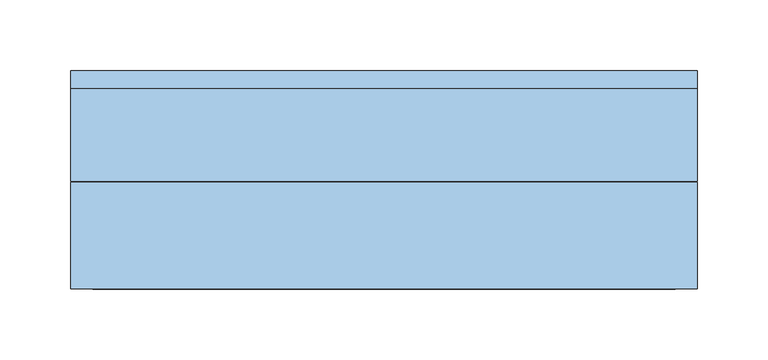
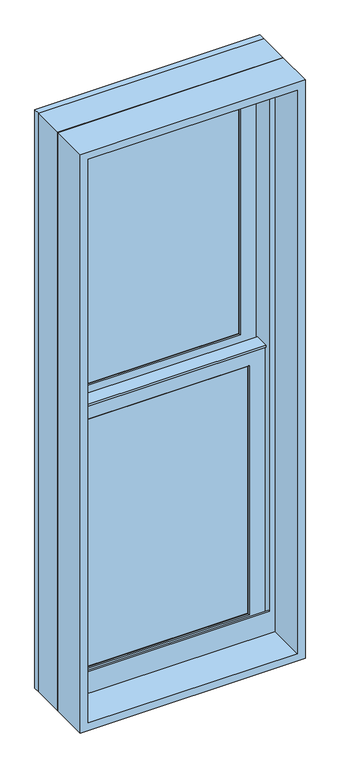
"""IFC4 building model written with IfcOpenShell, lengths in millimetres: window geometry, Window-Double_Hung-Marvin-Essential : ESDH1640."""

from ifc_helpers import new_model, si_unit, frame, origin, place, context, project, spatial, polyline, outline, extrude, faceted_brep, source, transform, mapped, element, save


def window_cbfb7004(model_context):
    return source(origin(), model_context, "Body", "SolidModel", [
        extrude(outline(polyline([(64.5583333, 20.6375), (64.5583333, 15.875), (45.5083333, 15.875), (45.5083333, 20.6375), (64.5583333, 20.6375)])), frame((0.0, 0.0, 1289.05), z_axis=(0.0, 0.0, 1.0), x_axis=(1.0, 0.0, 0.0)), (0.0, 0.0, 1.0), 527.05),
        extrude(outline(polyline([(-45.5083333, 20.6375), (-45.5083333, 15.875), (-64.5583333, 15.875), (-64.5583333, 20.6375), (-45.5083333, 20.6375)])), frame((0.0, 0.0, 1289.05), z_axis=(0.0, 0.0, 1.0), x_axis=(1.0, 0.0, 0.0)), (0.0, 0.0, 1.0), 527.05),
        extrude(outline(polyline([(165.1, 20.6375), (165.1, 15.875), (-165.1, 15.875), (-165.1, 20.6375), (165.1, 20.6375)])), frame((0.0, 0.0, 1543.05), z_axis=(0.0, 0.0, 1.0), x_axis=(1.0, 0.0, 0.0)), (0.0, 0.0, 1.0), 19.05),
        extrude(outline(polyline([(-64.5583333, 46.83125), (-64.5583333, 51.59375), (-45.5083333, 51.59375), (-45.5083333, 46.83125), (-64.5583333, 46.83125)])), frame((0.0, 0.0, 1854.2), z_axis=(0.0, 0.0, 1.0), x_axis=(1.0, 0.0, 0.0)), (0.0, 0.0, 1.0), 527.05),
        extrude(outline(polyline([(45.5083333, 46.83125), (45.5083333, 51.59375), (64.5583333, 51.59375), (64.5583333, 46.83125), (45.5083333, 46.83125)])), frame((0.0, 0.0, 1854.2), z_axis=(0.0, 0.0, 1.0), x_axis=(1.0, 0.0, 0.0)), (0.0, 0.0, 1.0), 527.05),
        extrude(outline(polyline([(-165.1, 46.83125), (-165.1, 51.59375), (165.1, 51.59375), (165.1, 46.83125), (-165.1, 46.83125)])), frame((0.0, 0.0, 2108.2), z_axis=(0.0, 0.0, 1.0), x_axis=(1.0, 0.0, 0.0)), (0.0, 0.0, 1.0), 19.05),
        extrude(outline(polyline([(64.5583333, 20.6375), (45.5083333, 20.6375), (45.5083333, 25.4), (64.5583333, 25.4), (64.5583333, 20.6375)])), frame((0.0, 0.0, 1289.05), z_axis=(0.0, 0.0, 1.0), x_axis=(1.0, 0.0, 0.0)), (0.0, 0.0, 1.0), 527.05),
        extrude(outline(polyline([(-45.5083333, 20.6375), (-64.5583333, 20.6375), (-64.5583333, 25.4), (-45.5083333, 25.4), (-45.5083333, 20.6375)])), frame((0.0, 0.0, 1289.05), z_axis=(0.0, 0.0, 1.0), x_axis=(1.0, 0.0, 0.0)), (0.0, 0.0, 1.0), 527.05),
        extrude(outline(polyline([(165.1, 20.6375), (-165.1, 20.6375), (-165.1, 25.4), (165.1, 25.4), (165.1, 20.6375)])), frame((0.0, 0.0, 1543.05), z_axis=(0.0, 0.0, 1.0), x_axis=(1.0, 0.0, 0.0)), (0.0, 0.0, 1.0), 19.05),
        extrude(outline(polyline([(-64.5583333, 56.35625), (-45.5083333, 56.35625), (-45.5083333, 51.59375), (-64.5583333, 51.59375), (-64.5583333, 56.35625)])), frame((0.0, 0.0, 1854.2), z_axis=(0.0, 0.0, 1.0), x_axis=(1.0, 0.0, 0.0)), (0.0, 0.0, 1.0), 527.05),
        extrude(outline(polyline([(45.5083333, 56.35625), (64.5583333, 56.35625), (64.5583333, 51.59375), (45.5083333, 51.59375), (45.5083333, 56.35625)])), frame((0.0, 0.0, 1854.2), z_axis=(0.0, 0.0, 1.0), x_axis=(1.0, 0.0, 0.0)), (0.0, 0.0, 1.0), 527.05),
        extrude(outline(polyline([(-165.1, 56.35625), (165.1, 56.35625), (165.1, 51.59375), (-165.1, 51.59375), (-165.1, 56.35625)])), frame((0.0, 0.0, 2108.2), z_axis=(0.0, 0.0, 1.0), x_axis=(1.0, 0.0, 0.0)), (0.0, 0.0, 1.0), 19.05),
        faceted_brep([(-192.0875, 5.6780605, 1846.1351748), (-192.0875, 5.6780605, 1841.5), (192.0875, 5.6780605, 1841.5), (192.0875, 5.6780605, 1846.1351748), (-192.0875, 34.8118605, 1846.1351748), (192.0875, 34.8118605, 1846.1351748), (192.0875, 34.8118605, 1841.5), (-192.0875, 34.8118605, 1841.5), (-192.0875, 30.1625, 1841.5), (-192.0875, 30.1625, 1262.0625), (-192.0875, 8.9241104, 1262.0625), (-192.0875, 8.9241104, 1841.5), (192.0875, 8.9241104, 1841.5), (192.0875, 30.1625, 1841.5), (192.0875, 8.9241104, 1262.0625), (192.0875, 30.1625, 1262.0625), (-176.2034752, 11.90625, 1827.2034752), (-176.2034752, 30.1625, 1827.2034752), (176.2034752, 30.1625, 1827.2034752), (176.2034752, 11.90625, 1827.2034752), (-159.54375, 10.4662439, 1810.54375), (-159.54375, 11.90625, 1810.54375), (159.54375, 11.90625, 1810.54375), (159.54375, 10.4662439, 1810.54375), (161.0858834, 8.9241104, 1812.0858834), (-161.0858834, 8.9241104, 1812.0858834), (176.2034752, 30.1625, 1277.9465248), (176.2034752, 11.90625, 1277.9465248), (159.54375, 11.90625, 1294.60625), (159.54375, 10.4662439, 1294.60625), (161.0858834, 8.9241104, 1293.0641166), (-176.2034752, 30.1625, 1277.9465248), (-176.2034752, 11.90625, 1277.9465248), (-159.54375, 11.90625, 1294.60625), (-159.54375, 10.4662439, 1294.60625), (-161.0858834, 8.9241104, 1293.0641166)], [[[0, 1, 2, 3]], [[4, 5, 6, 7]], [[1, 0, 4, 7, 8, 9, 10, 11]], [[2, 1, 11, 12]], [[7, 6, 13, 8]], [[3, 2, 12, 14, 15, 13, 6, 5]], [[0, 3, 5, 4]], [[16, 17, 18, 19]], [[20, 21, 22, 23]], [[20, 23, 24, 25]], [[19, 18, 26, 27]], [[23, 22, 28, 29]], [[24, 23, 29, 30]], [[27, 26, 31, 32]], [[29, 28, 33, 34]], [[30, 29, 34, 35]], [[15, 14, 10, 9]], [[15, 9, 8, 13], [18, 17, 31, 26]], [[17, 16, 32, 31]], [[16, 19, 27, 32], [22, 21, 33, 28]], [[21, 20, 34, 33]], [[20, 25, 35, 34]], [[10, 14, 12, 11], [25, 24, 30, 35]]]),
        extrude(outline(polyline([(38.5955581, 1827.2125), (33.5778968, 1827.2125), (33.5778968, 1828.8), (39.9405976, 1828.8), (39.9405976, 1827.2125), (61.515625, 1827.2125), (47.6307501, 1823.8975159), (38.5955581, 1823.8975159), (38.5955581, 1827.2125)])), frame((-192.0875, 0.0, 0.0), z_axis=(1.0, 0.0, 0.0), x_axis=(0.0, 1.0, 0.0)), (0.0, 0.0, 1.0), 384.175),
        faceted_brep([(222.25, 0.0, 1231.9), (222.25, 0.0, 2438.4), (-222.25, 0.0, 2438.4), (-222.25, 0.0, 1231.9), (196.05625, 0.0, 1293.01875), (-196.05625, 0.0, 1293.01875), (-196.05625, 0.0, 2412.20625), (196.05625, 0.0, 2412.20625), (196.05625, 3.96875, 1231.9), (-196.05625, 3.96875, 1231.9), (-196.05625, 3.96875, 1293.01875), (196.05625, 3.96875, 1293.01875), (-222.25, 65.6828125, 1231.9), (-196.05625, 65.6828125, 1231.9), (196.05625, 65.6828125, 1231.9), (222.25, 65.6828125, 1231.9), (-222.25, 65.6828125, 2438.4), (222.25, 65.6828125, 2438.4), (196.05625, 65.6828125, 2412.20625), (-196.05625, 65.6828125, 2412.20625)], [[[0, 1, 2, 3], [4, 5, 6, 7]], [[8, 9, 10, 11]], [[5, 4, 11, 10]], [[0, 3, 12, 13, 9, 8, 14, 15]], [[13, 12, 16, 17, 15, 14, 18, 19]], [[13, 19, 6, 5, 10, 9]], [[7, 6, 19, 18]], [[18, 14, 8, 11, 4, 7]], [[1, 0, 15, 17]], [[2, 1, 17, 16]], [[3, 2, 16, 12]]]),
        faceted_brep([(196.05625, 30.1625, 1835.15), (194.46875, 30.1625, 1835.15), (194.46875, 30.1625, 1256.2544613), (196.05625, 30.1625, 1256.2544613), (-194.46875, 30.1625, 1835.15), (-196.05625, 30.1625, 1835.15), (-196.05625, 30.1625, 1256.2544613), (-194.46875, 30.1625, 1256.2544613), (194.46875, 63.5, 1835.15), (196.05625, 63.5, 1835.15), (196.05625, 63.5, 1249.7743077), (194.46875, 63.5, 1249.7743077), (-196.05625, 63.5, 1835.15), (-194.46875, 63.5, 1835.15), (-194.46875, 63.5, 1249.7743077), (-196.05625, 63.5, 1249.7743077), (207.3108932, 3.96875, 1261.3460105), (207.3108932, 3.96875, 1231.9), (207.3108932, 65.6828125, 1231.9), (207.3108932, 65.6828125, 1249.350012), (-207.3108932, 3.96875, 1231.9), (-207.3108932, 3.96875, 1261.3460105), (-207.3108932, 65.6828125, 1249.350012), (-207.3108932, 65.6828125, 1231.9), (207.3108932, 78.58125, 1246.8428097), (-207.3108932, 78.58125, 1246.8428097), (-205.2971252, 68.2348864, 1248.8539391), (-187.33135, 68.2348864, 1248.8539391), (-187.33135, 65.6828125, 1249.350012), (187.33135, 65.6828125, 1249.350012), (187.33135, 68.2348864, 1248.8539391), (205.2971252, 68.2348864, 1248.8539391), (-222.25, 65.6828125, 1231.9), (-222.25, 78.5948249, 1231.9), (222.25, 78.5948249, 1231.9), (222.25, 65.6828125, 1231.9), (-222.25, 78.58125, 2438.4), (222.25, 78.58125, 2438.4), (207.3108932, 78.58125, 2423.4608932), (-207.3108932, 78.58125, 2423.4608932), (-222.25, 65.6828125, 2438.4), (-205.2971252, 68.2348864, 2421.4471252), (205.2971252, 68.2348864, 2421.4471252), (187.33135, 68.2348864, 2403.48135), (-187.33135, 68.2348864, 2403.48135), (-187.33135, 65.6828125, 2403.48135), (187.33135, 65.6828125, 2403.48135), (222.25, 65.6828125, 2438.4)], [[[0, 1, 2, 3]], [[4, 5, 6, 7]], [[8, 9, 10, 11]], [[12, 13, 14, 15]], [[1, 8, 11, 2]], [[9, 0, 3, 10]], [[1, 0, 9, 8]], [[5, 4, 13, 12]], [[5, 12, 15, 6]], [[13, 4, 7, 14]], [[16, 17, 18, 19]], [[20, 21, 22, 23]], [[24, 25, 26, 27, 28, 22, 21, 16, 19, 29, 30, 31], [3, 2, 11, 10], [7, 6, 15, 14]], [[17, 16, 21, 20]], [[17, 20, 23, 32, 33, 34, 35, 18]], [[34, 33, 36, 37], [25, 24, 38, 39]], [[33, 32, 40, 36]], [[39, 41, 26, 25]], [[41, 42, 31, 30, 43, 44, 27, 26]], [[44, 45, 28, 27]], [[40, 32, 23, 22, 28, 45, 46, 29, 19, 18, 35, 47]], [[36, 40, 47, 37]], [[39, 38, 42, 41]], [[44, 43, 46, 45]], [[34, 37, 47, 35]], [[42, 38, 24, 31]], [[46, 43, 30, 29]]]),
        extrude(outline(polyline([(172.24375, 11.90625), (-172.24375, 11.90625), (-172.24375, 15.08125), (172.24375, 15.08125), (172.24375, 11.90625)])), frame((0.0, 0.0, 1281.90625), z_axis=(0.0, 0.0, 1.0), x_axis=(1.0, 0.0, 0.0)), (0.0, 0.0, 1.0), 541.3375),
        extrude(outline(polyline([(172.24375, 42.8625), (-172.24375, 42.8625), (-172.24375, 46.0375), (172.24375, 46.0375), (172.24375, 42.8625)])), frame((0.0, 0.0, 1847.05625), z_axis=(0.0, 0.0, 1.0), x_axis=(1.0, 0.0, 0.0)), (0.0, 0.0, 1.0), 541.3375),
        faceted_brep([(-159.54375, 31.194477, 1810.54375), (-161.0858834, 32.7366104, 1812.0858834), (161.0858834, 32.7366104, 1812.0858834), (159.54375, 31.194477, 1810.54375), (-159.54375, 30.1625, 1810.54375), (159.54375, 30.1625, 1810.54375), (-192.0875, 32.7366104, 1843.0875), (-192.0875, 30.1625, 1843.0875), (192.0875, 30.1625, 1843.0875), (192.0875, 32.7366104, 1843.0875), (161.0858834, 32.7366104, 1293.0641166), (159.54375, 31.194477, 1294.60625), (159.54375, 30.1625, 1294.60625), (192.0875, 30.1625, 1262.0625), (192.0875, 32.7366104, 1262.0625), (-161.0858834, 32.7366104, 1293.0641166), (-159.54375, 31.194477, 1294.60625), (-159.54375, 30.1625, 1294.60625), (-192.0875, 30.1625, 1262.0625), (-192.0875, 32.7366104, 1262.0625)], [[[0, 1, 2, 3]], [[4, 0, 3, 5]], [[6, 7, 8, 9]], [[3, 2, 10, 11]], [[5, 3, 11, 12]], [[9, 8, 13, 14]], [[11, 10, 15, 16]], [[12, 11, 16, 17]], [[14, 13, 18, 19]], [[9, 14, 19, 6], [1, 15, 10, 2]], [[16, 15, 1, 0]], [[17, 16, 0, 4]], [[7, 18, 13, 8], [5, 12, 17, 4]], [[19, 18, 7, 6]]]),
        faceted_brep([(-176.2034752, 42.8625, 2392.3534752), (-176.2034752, 61.11875, 2392.3534752), (176.2034752, 61.11875, 2392.3534752), (176.2034752, 42.8625, 2392.3534752), (-159.54375, 41.4224939, 2375.69375), (-159.54375, 42.8625, 2375.69375), (159.54375, 42.8625, 2375.69375), (159.54375, 41.4224939, 2375.69375), (-161.0858834, 39.8803604, 2377.2358834), (161.0858834, 39.8803604, 2377.2358834), (-192.0875, 61.11875, 2408.2375), (-192.0875, 39.8803604, 2408.2375), (192.0875, 39.8803604, 2408.2375), (192.0875, 61.11875, 2408.2375), (176.2034752, 61.11875, 1843.0965248), (176.2034752, 42.8625, 1843.0965248), (159.54375, 42.8625, 1859.75625), (159.54375, 41.4224939, 1859.75625), (161.0858834, 39.8803604, 1858.2141166), (192.0875, 39.8803604, 1827.2125), (192.0875, 61.11875, 1827.2125), (-176.2034752, 61.11875, 1843.0965248), (-176.2034752, 42.8625, 1843.0965248), (-159.54375, 42.8625, 1859.75625), (-159.54375, 41.4224939, 1859.75625), (-161.0858834, 39.8803604, 1858.2141166), (-192.0875, 39.8803604, 1827.2125), (-192.0875, 61.11875, 1827.2125)], [[[0, 1, 2, 3]], [[4, 5, 6, 7]], [[8, 4, 7, 9]], [[10, 11, 12, 13]], [[3, 2, 14, 15]], [[7, 6, 16, 17]], [[9, 7, 17, 18]], [[13, 12, 19, 20]], [[15, 14, 21, 22]], [[17, 16, 23, 24]], [[18, 17, 24, 25]], [[20, 19, 26, 27]], [[13, 20, 27, 10], [1, 21, 14, 2]], [[22, 21, 1, 0]], [[3, 15, 22, 0], [5, 23, 16, 6]], [[24, 23, 5, 4]], [[25, 24, 4, 8]], [[11, 26, 19, 12], [9, 18, 25, 8]], [[27, 26, 11, 10]]]),
        faceted_brep([(-192.0875, 61.11875, 1827.2125), (-192.0875, 63.6928604, 1827.2125), (192.0875, 63.6928604, 1827.2125), (192.0875, 61.11875, 1827.2125), (-159.54375, 62.150727, 1859.75625), (-159.54375, 61.11875, 1859.75625), (159.54375, 61.11875, 1859.75625), (159.54375, 62.150727, 1859.75625), (-161.0858834, 63.6928604, 1858.2141166), (161.0858834, 63.6928604, 1858.2141166), (192.0875, 63.6928604, 2408.2375), (192.0875, 61.11875, 2408.2375), (159.54375, 61.11875, 2375.69375), (159.54375, 62.150727, 2375.69375), (161.0858834, 63.6928604, 2377.2358834), (-192.0875, 63.6928604, 2408.2375), (-192.0875, 61.11875, 2408.2375), (-159.54375, 61.11875, 2375.69375), (-159.54375, 62.150727, 2375.69375), (-161.0858834, 63.6928604, 2377.2358834)], [[[0, 1, 2, 3]], [[4, 5, 6, 7]], [[8, 4, 7, 9]], [[3, 2, 10, 11]], [[7, 6, 12, 13]], [[9, 7, 13, 14]], [[11, 10, 15, 16]], [[13, 12, 17, 18]], [[14, 13, 18, 19]], [[16, 15, 1, 0]], [[3, 11, 16, 0], [5, 17, 12, 6]], [[18, 17, 5, 4]], [[19, 18, 4, 8]], [[1, 15, 10, 2], [9, 14, 19, 8]]]),
        extrude(outline(polyline([(172.24375, 26.19375), (-172.24375, 26.19375), (-172.24375, 30.1625), (172.24375, 30.1625), (172.24375, 26.19375)])), frame((0.0, 0.0, 1281.90625), z_axis=(0.0, 0.0, 1.0), x_axis=(1.0, 0.0, 0.0)), (0.0, 0.0, 1.0), 541.3375),
        extrude(outline(polyline([(172.24375, 57.15), (-172.24375, 57.15), (-172.24375, 61.11875), (172.24375, 61.11875), (172.24375, 57.15)])), frame((0.0, 0.0, 1847.05625), z_axis=(0.0, 0.0, 1.0), x_axis=(1.0, 0.0, 0.0)), (0.0, 0.0, 1.0), 541.3375),
        extrude(outline(polyline([(2438.4, 222.25), (2438.4, -222.25), (1231.9, -222.25), (1231.9, 222.25), (2438.4, 222.25)]), holes=[polyline([(2422.525, 206.375), (1247.775, 206.375), (1247.775, -206.375), (2422.525, -206.375), (2422.525, 206.375)])]), frame((0.0, -76.2, 0.0), z_axis=(0.0, 1.0, 0.0), x_axis=(0.0, 0.0, 1.0)), (0.0, 0.0, 1.0), 75.40625),
    ])


if __name__ == "__main__":
    model = new_model("IFC4")
    model_context = context("Model", 3, world=origin())
    ifc_project = project(units=[si_unit("LENGTHUNIT", "METRE", prefix="MILLI")], contexts=[model_context])
    site = spatial("IfcSite", under=ifc_project)
    building = spatial("IfcBuilding", under=site)
    placement = place(None, origin())
    window_shape = window_cbfb7004(model_context)
    element("IfcWindow", 1, ObjectType="Window-Double_Hung-Marvin-Essential : ESDH1640", at=placement, inside=building, context=model_context, shape_type="MappedRepresentation", body=[
        mapped(window_shape, transform((0.0, 0.0, 0.0), x_axis=(1.0, 0.0, 0.0), y_axis=(0.0, 1.0, 0.0), z_axis=(0.0, 0.0, 1.0))),
    ])
    save(model, "model.ifc")

# Revit data of these elements
# Type "Window-Double_Hung-Marvin-Essential : ESDH1640"
#   Type Mark = "47"
#   Window Type = "Essential Double Hung"
#   Product data url = "https://bimobject.com/marvin-windows-and-doors/product/marvin-dhwau"
#   Product Guid = "c4a96547-874c-4385-91dc-a058adc19d98"
#   Frame = "All Ultrex"
#   Egress Window = "No"
#   URL = "www.marvin.com"
#   Model = "ESDH1640"
#   Manufacturer = "Marvin Windows and Doors"
#   Label Egress = ""
#   Glass Type = "IG Low E II with Argon"
#   Design Pressure = "DP50"
#   Description = "1848 DBHG"
#   Analytic Construction = "<None>"
#   Prairie Corner Width = 0' - 4"
#   Prairie Corner Height = 0' - 4"
#   Egress Width = 1' - 2 9/16"
#   Egress Height = 1' - 7 27/128"
#   Rough Width = 1' - 6"
#   Rough Height = 4' - 0"
#   Nominal Width = 1' - 6"
#   Nominal Height = 4' - 0"
#   Inset to Installation Flange [instance default] = 0' - 1"
#   Height = 3' - 11 1/2"
#   Egress Area = 1.94277 SF
#   Default Head Height = 8' - 0"
#   Width = 1' - 5 1/2"
#   Daylight Area = 3.54411 SF
#   DLO Width = 1' - 0 9/16"
#   DLO Height = 1' - 8 5/16"
#   Muntins Top Sash = yes
#   Lites Wide Top Sash = 3
#   Lites Wide Bottom Sash = 3
#   Lites High Top Sash = 2
#   Lites High Bottom Sash = 2
#   Lite Cut Prairie 9 = no
#   Lite Cut HV Grid = yes
#   Muntins Bottom Sash = yes
#   Label Visibility = no
#   Jamb Extension Visibility = yes
#   Edition number = 1
#   Interior Material = Ultrex-Marvin-Stonewhite
#   Glazing Material = Glass-Marvin-IG Low E II with Argon
#   Cladding Material = Ultrex-Marvin-Pebblegray
#   Wall Closure = (empty or 0)
#   Assembly Code = ""
# Element 1 (IfcWindow, "Window-Double_Hung-Marvin-Essential : ESDH1640")
#   Materials on its faces: "Ultrex-Marvin-Pebblegray", "Ultrex-Marvin-Stonewhite", "Glass-Marvin-IG Low E II with Argon"
# Materials
#   "Ultrex-Marvin-Stonewhite": class "Paint", colour RGB 250 251 245, transparency 0
#   "Glass-Marvin-IG Low E II with Argon": class "Glass", colour RGB 0 128 192, transparency 0.85
#   "Ultrex-Marvin-Pebblegray": class "Paint", colour RGB 189 185 173, transparency 0
